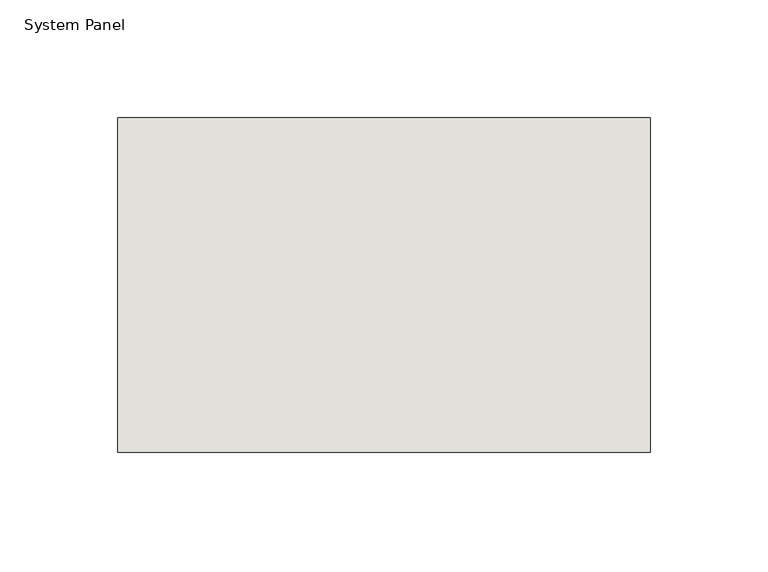
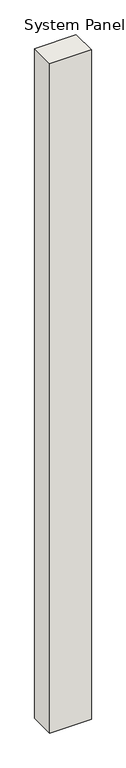
"""IFC4 building model written with IfcOpenShell, lengths in millimetres: wall geometry, System Panel : NLRS_21_CWP_hsb-vulling minerale wol 142 _gen_rsf."""

from ifc_helpers import new_model, si_unit, origin, origin_with_axes, place, context, project, spatial, polyline, outline, extrude, source, transform, mapped, element, save


def system_panel_6e26c10f(model_context):
    return source(origin(), model_context, "Body", "SweptSolid", [
        extrude(outline(polyline([(113.0000002, -71.0), (-113.0000002, -71.0), (-113.0000002, 71.0), (113.0000002, 71.0), (113.0000002, -71.0)])), origin_with_axes(), (0.0, 0.0, 1.0), 3849.0),
    ])


if __name__ == "__main__":
    model = new_model("IFC4")
    model_context = context("Model", 3, world=origin())
    ifc_project = project(units=[si_unit("LENGTHUNIT", "METRE", prefix="MILLI")], contexts=[model_context])
    site = spatial("IfcSite", under=ifc_project)
    building = spatial("IfcBuilding", under=site)
    placement = place(None, origin())
    system_panel_shape = system_panel_6e26c10f(model_context)
    element("IfcWall", 1, ObjectType="System Panel : NLRS_21_CWP_hsb-vulling minerale wol 142 _gen_rsf", at=placement, inside=building, context=model_context, shape_type="MappedRepresentation", body=[
        mapped(system_panel_shape, transform((0.0, 0.0, 0.0), x_axis=(1.0, 0.0, 0.0), y_axis=(0.0, 1.0, 0.0), z_axis=(0.0, 0.0, 1.0))),
    ])
    save(model, "model.ifc")

# Revit data of these elements
# Type "System Panel : NLRS_21_CWP_hsb-vulling minerale wol 142 _gen_rsf"
#   Type IfcGUID = "07M7mRoiH1CR8m_RSKIwpC"
#   Assembly Code = "21.23"
#   IfcExportAs = "IfcWall"
# Element 1 (IfcWall, "System Panel : NLRS_21_CWP_hsb-vulling minerale wol 142 _gen_rsf")
#   Materials on its faces: "NLRS_m1_isolatie minerale wol_gen_rsf"
# Materials
#   "NLRS_m1_isolatie minerale wol_gen_rsf": class "M - Anorganische materialen", colour RGB 200 200 140, transparency 0, Keynote = "m1", Manufacturer = "Revit Standards Foundation", URL = "www.revitstandards.org", Description = "isolatie minerale wol", Cost = 0
